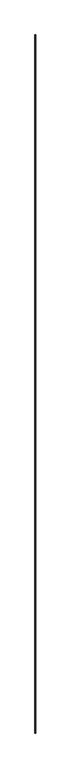
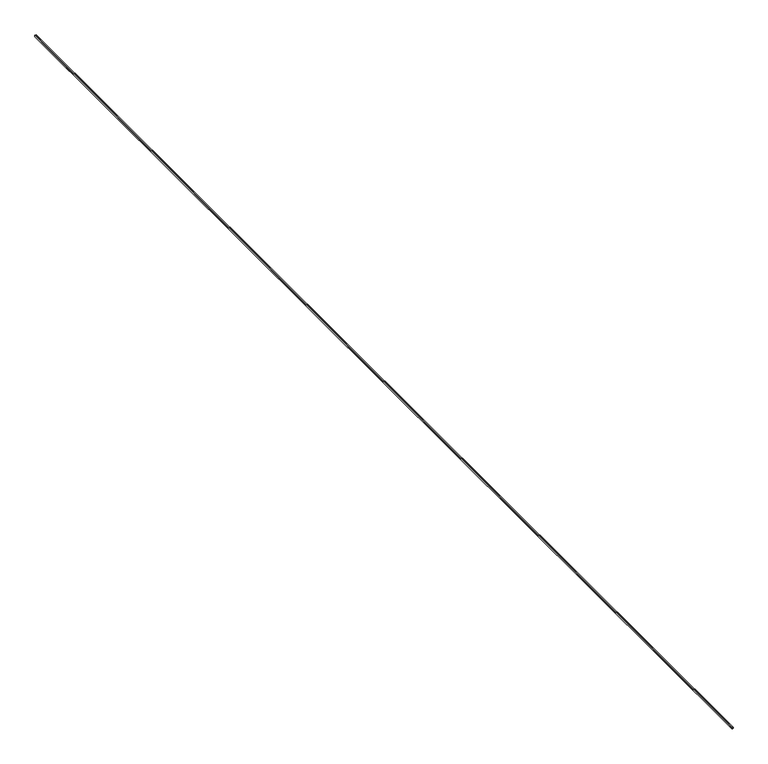
"""IFC4 building model written with IfcOpenShell, lengths in millimetres: proxy geometry, Inner panel:Inner panel:1:Inner panel:1 : Inner panel:Inner panel:300324:2:Inner panel:1:Inner panel:1 : Inner panel:Inner panel:300324:2 : Inner panel:Inner panel:1:Inner panel:1 : Inner panel:Inner panel:300324:300043:59 : Inner panel:Inner panel:1:Inner panel:1 : Inner panel:Inner panel:300324:2:Inner panel:1:Inner panel:1 : Inner panel:Inner panel:300324:2 : Inner panel:Inner panel:1:Inner panel:1 : Inner panel:Inner panel:300324:300043:308120."""

from ifc_helpers import new_model, si_unit, frame, origin, place, context, project, spatial, polyline, outline, extrude, source, transform, mapped, element, save


def generic_models_3de8d47e(model_context):
    return source(origin(), model_context, "Body", "SweptSolid", [
        extrude(outline(polyline([(3882.914021, 558758.0377931), (3880.5348354, 558758.1369258), (3881.1957202, 558773.9981633), (3847.8871214, 558775.3860216), (3846.4992631, 558742.0774228), (3879.807862, 558740.6895645), (3880.4687469, 558756.550802), (3882.8479325, 558756.4516693), (3882.0879149, 558738.2112461), (3844.0209448, 558739.7973699), (3845.6070685, 558777.86434), (3883.6740386, 558776.2782162), (3882.914021, 558758.0377931)])), frame((0.0, -579337.5059673, 0.0), z_axis=(0.0, 1.0, 0.0), x_axis=(0.0, 0.0, 1.0)), (0.0, 0.0, 1.0), 33093.2895833),
    ])


if __name__ == "__main__":
    model = new_model("IFC4")
    model_context = context("Model", 3, world=origin())
    ifc_project = project(units=[si_unit("LENGTHUNIT", "METRE", prefix="MILLI")], contexts=[model_context])
    site = spatial("IfcSite", under=ifc_project)
    building = spatial("IfcBuilding", under=site)
    placement = place(None, origin())
    generic_models_shape = generic_models_3de8d47e(model_context)
    element("IfcBuildingElementProxy", 1, Name="Inner panel:Inner panel:1:Inner panel:1 : Inner panel:Inner panel:300324:2:Inner panel:1:Inner panel:1 : Inner panel:Inner panel:300324:2 : Inner panel:Inner panel:1:Inner panel:1 : Inner panel:Inner panel:300324:300043:59 : Inner panel:Inner panel:1:Inner panel:1 : Inner panel:Inner panel:300324:2:Inner panel:1:Inner panel:1 : Inner panel:Inner panel:300324:2 : Inner panel:Inner panel:1:Inner panel:1 : Inner panel:Inner panel:300324:300043:308120", ObjectType="Inner panel:Inner panel:1:Inner panel:1 : Inner panel:Inner panel:300324:2:Inner panel:1:Inner panel:1 : Inner panel:Inner panel:300324:2 : Inner panel:Inner panel:1:Inner panel:1 : Inner panel:Inner panel:300324:300043:59 : Inner panel:Inner panel:1:Inner panel:1 : Inner panel:Inner panel:300324:2:Inner panel:1:Inner panel:1 : Inner panel:Inner panel:300324:2 : Inner panel:Inner panel:1:Inner panel:1 : Inner panel:Inner panel:300324:300043:308120", at=placement, inside=building, context=model_context, shape_type="MappedRepresentation", body=[
        mapped(generic_models_shape, transform((0.0, 0.0, 0.0), x_axis=(1.0, 0.0, 0.0), y_axis=(0.0, 1.0, 0.0), z_axis=(0.0, 0.0, 1.0))),
    ])
    save(model, "model.ifc")

# Revit data of these elements
# Type "Inner panel:Inner panel:1:Inner panel:1 : Inner panel:Inner panel:300324:2:Inner panel:1:Inner panel:1 : Inner panel:Inner panel:300324:2 : Inner panel:Inner panel:1:Inner panel:1 : Inner panel:Inner panel:300324:300043:59 : Inner panel:Inner panel:1:Inner panel:1 : Inner panel:Inner panel:300324:2:Inner panel:1:Inner panel:1 : Inner panel:Inner panel:300324:2 : Inner panel:Inner panel:1:Inner panel:1 : Inner panel:Inner panel:300324:300043:308120"
#   NameOverride = "Inner panel:Inner panel:1:Inner panel:1 : Inner panel:Inner panel:300324:2:Inner panel:1:Inner panel:1 : Inner panel:Inner panel:300324:2 : Inner panel:Inner panel:1:Inner panel:1 : Inner panel:Inner panel:300324:300043:308120"
#   ObjectTypeOverride = "Inner panel:1:Inner panel:1 : Inner panel:Inner panel:300324:2 : Inner panel:Inner panel:1:Inner panel:1 : Inner panel:Inner panel:300324:300043"
#   Reference = "Inner panel"
#   Tag = "308120"
# Element 1 (IfcBuildingElementProxy, "Inner panel:Inner panel:1:Inner panel:1 : Inner panel:Inner panel:300324:2:Inner panel:1:Inner panel:1 : Inner panel:Inner panel:300324:2 : Inner panel:Inner panel:1:Inner panel:1 : Inner panel:Inner panel:300324:300043:59 : Inner panel:Inner panel:1:Inner panel:1 : Inner panel:Inner panel:300324:2:Inner panel:1:Inner panel:1 : Inner panel:Inner panel:300324:2 : Inner panel:Inner panel:1:Inner panel:1 : Inner panel:Inner panel:300324:300043:308120")
#   Materials on its faces: "1 1/2\" X 1 1/2\" SPLIT-SEAM SQUARE TUBING (~24\" CANTILEVER FROM C.L. OF GLULAM)"
# Materials
#   "1 1/2\" X 1 1/2\" SPLIT-SEAM SQUARE TUBING (~24\" CANTILEVER FROM C.L. OF GLULAM)": class "Unassigned", colour RGB 202 201 200, transparency 0, Cost = 0
